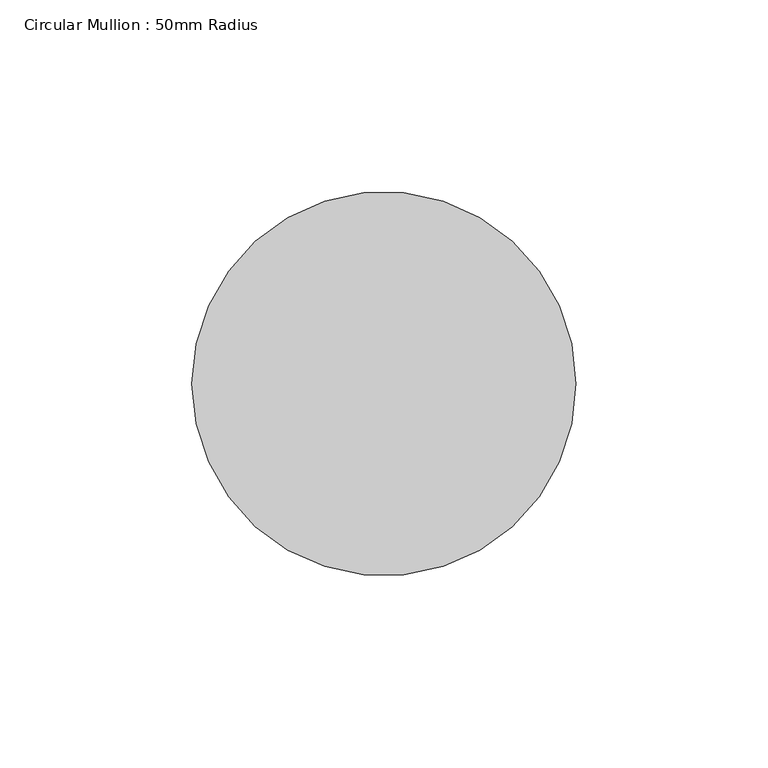
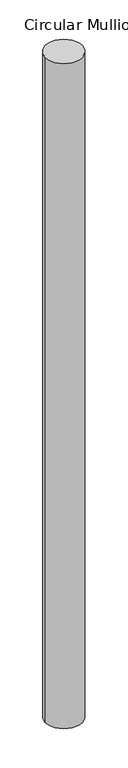
"""IFC4 building model written with IfcOpenShell, lengths in millimetres: member geometry, Circular Mullion : 50mm Radius."""

from ifc_helpers import new_model, si_unit, point, frame, frame_2d, origin, place, context, project, spatial, circle_curve, trimmed, segment, composite_curve, outline, extrude, source, transform, mapped, element, save


def circular_mullion_50mm_radius_ac8a11f8(model_context):
    return source(origin(), model_context, "Body", "SweptSolid", [
        extrude(outline(composite_curve([segment(trimmed(circle_curve(frame_2d((-50.0, 0.0)), 50.0), [point((0.0, 0.0))], [point((-100.0, 0.0))], False, "CARTESIAN"), True, "CONTINUOUS"), segment(trimmed(circle_curve(frame_2d((-50.0, 0.0)), 50.0), [point((-100.0, 0.0))], [point((0.0, 0.0))], False, "CARTESIAN"), True, "CONTINUOUS")], self_intersect=False)), frame((0.0, 0.0, -1919.922387), z_axis=(0.0, 0.0, 1.0), x_axis=(1.0, 0.0, 0.0)), (0.0, 0.0, 1.0), 1919.922387),
    ])


if __name__ == "__main__":
    model = new_model("IFC4")
    model_context = context("Model", 3, world=origin())
    ifc_project = project(units=[si_unit("LENGTHUNIT", "METRE", prefix="MILLI")], contexts=[model_context])
    site = spatial("IfcSite", under=ifc_project)
    building = spatial("IfcBuilding", under=site)
    placement = place(None, origin())
    circular_mullion_50mm_radius_shape = circular_mullion_50mm_radius_ac8a11f8(model_context)
    element("IfcMember", 1, ObjectType="Circular Mullion : 50mm Radius", at=placement, inside=building, context=model_context, shape_type="MappedRepresentation", body=[
        mapped(circular_mullion_50mm_radius_shape, transform((0.0, 0.0, 0.0), x_axis=(1.0, 0.0, 0.0), y_axis=(0.0, 1.0, 0.0), z_axis=(0.0, 0.0, 1.0))),
    ])
    save(model, "model.ifc")

# Revit data of these elements
# Type "Circular Mullion : 50mm Radius"
#   built-in parameter 1007350 = 0.164042 (stored number, unit not read)
# Element 1 (IfcMember, "Circular Mullion : 50mm Radius")
#   Materials on its faces: "Aluminium"
# Materials
#   "Aluminium": class "Metal", colour RGB 247 247 247, transparency 0, Description = "Aluminium 6061", Cost = 0
